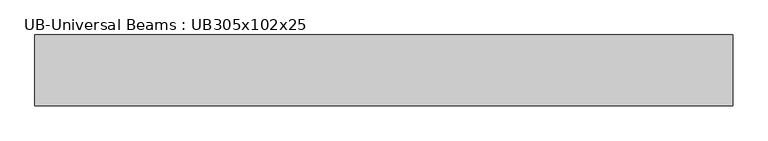
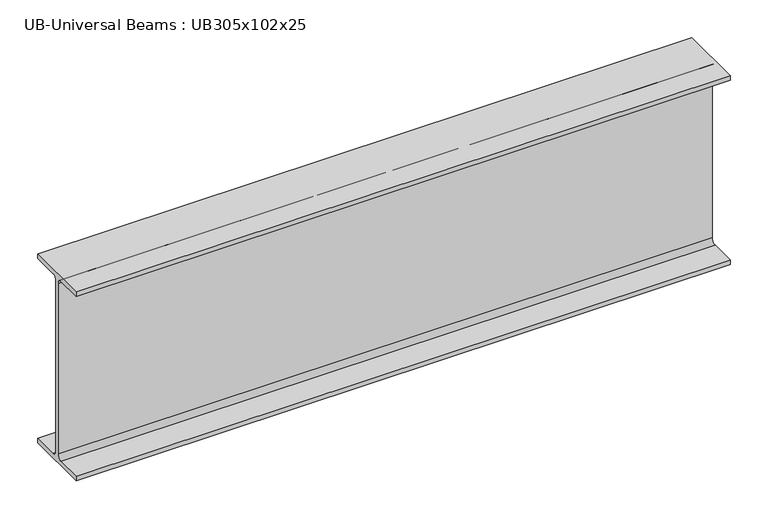
"""IFC4 building model written with IfcOpenShell, lengths in millimetres: beam geometry, UB-Universal Beams : UB305x102x25."""

import ifcopenshell
import ifcopenshell.guid

model = None  # the IFC model being written
_history = None  # IfcOwnerHistory: only IFC2X3 demands one
_inside = {}  # id of a spatial element -> (the spatial element, [elements in it])
_under = {}  # id of a project, library or spatial element -> (it, [spatial elements below it])
_declared = {}  # id of a project -> (the project, [libraries it declares])
_typed = {}  # id of a type object -> (the type object, [elements of that type])
_made_of = {}  # id of a material, layer set ... -> (it, [elements and type objects made of it])


def new_model(schema):
    """Start an empty IFC model of exactly this schema.

    Asked for "IFC4X3", IfcOpenShell would pick the latest addendum, in which some entities
    have other attributes; the version numbers below select the first issue.
    IFC2X3 requires an IfcOwnerHistory on every rooted entity: one is made here for all.
    """
    global model, _history
    if schema == "IFC4X3":
        model = ifcopenshell.file(schema_version=(4, 3, 0, 0))
    else:
        model = ifcopenshell.file(schema=schema)
    _inside.clear()
    _under.clear()
    _declared.clear()
    _typed.clear()
    _made_of.clear()
    _history = None
    if model.schema == "IFC2X3":
        org = make("IfcOrganization", Name="unknown")
        user = make(
            "IfcPersonAndOrganization",
            ThePerson=make("IfcPerson", FamilyName="unknown"),
            TheOrganization=org,
        )
        app = make(
            "IfcApplication",
            ApplicationDeveloper=org,
            Version="unknown",
            ApplicationFullName="unknown",
            ApplicationIdentifier="unknown",
        )
        _history = make(
            "IfcOwnerHistory",
            OwningUser=user,
            OwningApplication=app,
            ChangeAction="ADDED",
            CreationDate=0,
        )
    return model


def make(cls, **values):
    """One entity of the class cls with the attributes given. An attribute that is None is left unset."""
    return model.create_entity(
        cls, **{name: value for name, value in values.items() if value is not None}
    )


def rooted(cls, **values):
    """An entity with a GlobalId (a new one), such as an element, a storey or a relation."""
    return make(cls, GlobalId=ifcopenshell.guid.new(), OwnerHistory=_history, **values)


def si_unit(unit_type, name, prefix=None):
    """IfcSIUnit, for example si_unit("LENGTHUNIT", "METRE", prefix="MILLI")."""
    return make("IfcSIUnit", UnitType=unit_type, Prefix=prefix, Name=name)


def assignment(units):
    """IfcUnitAssignment: the units of a project."""
    return None if units is None else make("IfcUnitAssignment", Units=units)


def point(xyz):
    """IfcCartesianPoint."""
    return None if xyz is None else make("IfcCartesianPoint", Coordinates=xyz)


def direction(xyz):
    """IfcDirection."""
    return None if xyz is None else make("IfcDirection", DirectionRatios=xyz)


def frame(location, z_axis=None, x_axis=None):
    """IfcAxis2Placement3D, a coordinate frame: its origin and axes. An axis left out is left unset."""
    return make(
        "IfcAxis2Placement3D",
        Location=point(location),
        Axis=direction(z_axis),
        RefDirection=direction(x_axis),
    )


def frame_2d(location, x_axis=None):
    """IfcAxis2Placement2D, a coordinate frame in the plane: its origin and x axis."""
    return make(
        "IfcAxis2Placement2D", Location=point(location), RefDirection=direction(x_axis)
    )


def origin():
    """The frame at (0, 0, 0) with its axes left unset."""
    return frame((0.0, 0.0, 0.0))


def place(relative_to, where):
    """IfcLocalPlacement: puts the frame where relative to a parent placement (None: the world)."""
    return make(
        "IfcLocalPlacement", PlacementRelTo=relative_to, RelativePlacement=where
    )


def context(
    kind, dimensions, precision=None, world=None, true_north=None, identifier=None
):
    """IfcGeometricRepresentationContext, for example the 3D "Model" context."""
    return make(
        "IfcGeometricRepresentationContext",
        ContextIdentifier=identifier,
        ContextType=kind,
        CoordinateSpaceDimension=dimensions,
        Precision=precision,
        WorldCoordinateSystem=world,
        TrueNorth=true_north,
    )


def project(units=None, contexts=None):
    """IfcProject with its units and contexts."""
    return rooted(
        "IfcProject",
        Name="project",
        RepresentationContexts=contexts,
        UnitsInContext=assignment(units),
    )


def spatial(cls, under=None, at=None, **own):
    """A site, building, storey or space (cls), placed at a placement, below another one or the project."""
    s = rooted(cls, ObjectPlacement=at, **own)
    if under is not None:
        _under.setdefault(under.id(), (under, []))[1].append(s)
    return s


def polyline(points):
    """IfcPolyline through the points."""
    return make("IfcPolyline", Points=[point(p) for p in points])


def circle_curve(where, radius):
    """IfcCircle in the frame where."""
    return make("IfcCircle", Position=where, Radius=radius)


def trimmed(basis, trim1, trim2, sense, master):
    """IfcTrimmedCurve: the piece of a basis curve between two trims."""
    return make(
        "IfcTrimmedCurve",
        BasisCurve=basis,
        Trim1=trim1,
        Trim2=trim2,
        SenseAgreement=sense,
        MasterRepresentation=master,
    )


def segment(curve, same_sense, transition):
    """IfcCompositeCurveSegment."""
    return make(
        "IfcCompositeCurveSegment",
        Transition=transition,
        SameSense=same_sense,
        ParentCurve=curve,
    )


def composite_curve(segments, self_intersect=None):
    """IfcCompositeCurve: segments joined end to end."""
    return make("IfcCompositeCurve", Segments=segments, SelfIntersect=self_intersect)


def outline(outer, holes=None, kind="AREA"):
    """IfcArbitraryClosedProfileDef: a profile drawn as a closed curve; with holes, ...WithVoids."""
    if holes is None:
        return make("IfcArbitraryClosedProfileDef", ProfileType=kind, OuterCurve=outer)
    return make(
        "IfcArbitraryProfileDefWithVoids",
        ProfileType=kind,
        OuterCurve=outer,
        InnerCurves=holes,
    )


def extrude(swept, where, along, depth):
    """IfcExtrudedAreaSolid: the profile swept, set in the frame where, extruded along a direction by depth."""
    return make(
        "IfcExtrudedAreaSolid",
        SweptArea=swept,
        Position=where,
        ExtrudedDirection=direction(along),
        Depth=depth,
    )


def shape(context_of_items, identifier, shape_type, items):
    """IfcShapeRepresentation: the items that make up one representation, for example the "Body"."""
    return make(
        "IfcShapeRepresentation",
        ContextOfItems=context_of_items,
        RepresentationIdentifier=identifier,
        RepresentationType=shape_type,
        Items=items,
    )


def source(mapping_origin, context_of_items, identifier, shape_type, items):
    """IfcRepresentationMap: a shape defined once, which mapped items show again and again."""
    return make(
        "IfcRepresentationMap",
        MappingOrigin=mapping_origin,
        MappedRepresentation=shape(context_of_items, identifier, shape_type, items),
    )


def transform(
    local_origin,
    x_axis=None,
    y_axis=None,
    z_axis=None,
    scale=None,
    scale2=None,
    scale3=None,
    uniform=True,
):
    """IfcCartesianTransformationOperator3D, or its non-uniform kind. x_axis, y_axis, z_axis: its Axis1, 2, 3."""
    if uniform:
        return make(
            "IfcCartesianTransformationOperator3D",
            Axis1=direction(x_axis),
            Axis2=direction(y_axis),
            LocalOrigin=point(local_origin),
            Scale=scale,
            Axis3=direction(z_axis),
        )
    return make(
        "IfcCartesianTransformationOperator3DnonUniform",
        Axis1=direction(x_axis),
        Axis2=direction(y_axis),
        LocalOrigin=point(local_origin),
        Scale=scale,
        Axis3=direction(z_axis),
        Scale2=scale2,
        Scale3=scale3,
    )


def mapped(mapping_source, mapping_target):
    """IfcMappedItem: shows the shape of a source again, moved by a transform."""
    return make(
        "IfcMappedItem", MappingSource=mapping_source, MappingTarget=mapping_target
    )


def made_of(thing, what):
    """Note that an element or type object is made of a material, layer set ...; save() writes the relation."""
    if what is not None:
        _made_of.setdefault(what.id(), (what, []))[1].append(thing)
    return thing


def element(
    cls,
    number,
    at=None,
    inside=None,
    cuts=None,
    type_object=None,
    material=None,
    context=None,
    identifier="Body",
    shape_type=None,
    held_by="IfcProductDefinitionShape",
    body=None,
    shapes=None,
    **own,
):
    """One element of the class cls, such as IfcWall. Its Tag is "e" and its number.

    at: its placement. inside: the storey or other place that contains it. cuts: it is an
    opening in that element (IfcRelVoidsElement). A single representation is given by context,
    identifier, shape_type and body (its items); several are given by shapes. held_by: the class
    of the entity that holds the representations. save() writes the other relations.
    """
    e = rooted(cls, Tag="e%d" % number, ObjectPlacement=at, **own)
    if body is not None:
        shapes = [shape(context, identifier, shape_type, body)]
    if shapes is not None:
        e.Representation = make(held_by, Representations=shapes)
    if inside is not None:
        _inside.setdefault(inside.id(), (inside, []))[1].append(e)
    if cuts is not None:
        rooted(
            "IfcRelVoidsElement", RelatingBuildingElement=cuts, RelatedOpeningElement=e
        )
    if type_object is not None:
        _typed.setdefault(type_object.id(), (type_object, []))[1].append(e)
    return made_of(e, material)


def aggregate(whole, parts):
    """IfcRelAggregates: a whole, such as a stair, and the parts it consists of."""
    return rooted("IfcRelAggregates", RelatingObject=whole, RelatedObjects=parts)


def save(model, path):
    """Write the relations noted so far, then the file.

    IfcRelAggregates (storeys below a building ...), IfcRelContainedInSpatialStructure (elements
    in a storey), IfcRelDefinesByType, IfcRelAssociatesMaterial and IfcRelDeclares: one each for
    every whole, place, type object, material and project.
    """
    for whole, parts in _under.values():
        aggregate(whole, parts)
    for where, things in _inside.values():
        rooted(
            "IfcRelContainedInSpatialStructure",
            RelatedElements=things,
            RelatingStructure=where,
        )
    for kind, things in _typed.values():
        rooted("IfcRelDefinesByType", RelatedObjects=things, RelatingType=kind)
    for what, things in _made_of.values():
        rooted("IfcRelAssociatesMaterial", RelatedObjects=things, RelatingMaterial=what)
    for by, libraries in _declared.values():
        rooted("IfcRelDeclares", RelatingContext=by, RelatedDefinitions=libraries)
    model.write(path)


def ub_universal_beams_ub305x102x25_41277c4d(model_context):
    return source(origin(), model_context, "Body", "SweptSolid", [
        extrude(outline(composite_curve([segment(polyline([(50.8, -145.55), (50.8, -152.55), (-50.8, -152.55), (-50.8, -145.55), (-10.5, -145.55)]), True, "CONTINUOUS"), segment(trimmed(circle_curve(frame_2d((-10.5, -137.95)), 7.6), [point((-10.5, -145.55))], [point((-2.9, -137.95))], True, "CARTESIAN"), True, "CONTINUOUS"), segment(polyline([(-2.9, -137.95), (-2.9, 137.95)]), True, "CONTINUOUS"), segment(trimmed(circle_curve(frame_2d((-10.5, 137.95)), 7.6), [point((-2.9, 137.95))], [point((-10.5, 145.55))], True, "CARTESIAN"), True, "CONTINUOUS"), segment(polyline([(-10.5, 145.55), (-50.8, 145.55), (-50.8, 152.55), (50.8, 152.55), (50.8, 145.55), (10.5, 145.55)]), True, "CONTINUOUS"), segment(trimmed(circle_curve(frame_2d((10.5, 137.95)), 7.6), [point((10.5, 145.55))], [point((2.9, 137.95))], True, "CARTESIAN"), True, "CONTINUOUS"), segment(polyline([(2.9, 137.95), (2.9, -137.95)]), True, "CONTINUOUS"), segment(trimmed(circle_curve(frame_2d((10.5, -137.95)), 7.6), [point((2.9, -137.95))], [point((10.5, -145.55))], True, "CARTESIAN"), True, "CONTINUOUS"), segment(polyline([(10.5, -145.55), (50.8, -145.55)]), True, "CONTINUOUS")], self_intersect=False)), frame((-500.0, 0.0, 0.0), z_axis=(1.0, 0.0, 0.0), x_axis=(0.0, 1.0, 0.0)), (0.0, 0.0, 1.0), 1000.0),
    ])


if __name__ == "__main__":
    model = new_model("IFC4")
    model_context = context("Model", 3, world=origin())
    ifc_project = project(units=[si_unit("LENGTHUNIT", "METRE", prefix="MILLI")], contexts=[model_context])
    site = spatial("IfcSite", under=ifc_project)
    building = spatial("IfcBuilding", under=site)
    placement = place(None, origin())
    ub_universal_beams_ub305x102x25_shape = ub_universal_beams_ub305x102x25_41277c4d(model_context)
    element("IfcBeam", 1, ObjectType="UB-Universal Beams : UB305x102x25", at=placement, inside=building, context=model_context, shape_type="MappedRepresentation", body=[
        mapped(ub_universal_beams_ub305x102x25_shape, transform((0.0, 0.0, 0.0), x_axis=(1.0, 0.0, 0.0), y_axis=(0.0, 1.0, 0.0), z_axis=(0.0, 0.0, 1.0))),
    ])
    save(model, "model.ifc")

# Revit data of these elements
# Type "UB-Universal Beams : UB305x102x25"
#   Section Name Key = "UB305X102X25"
#   Width = 10.16 cm
#   Web Thickness = 0.58 cm
#   Web Fillet = 0.76 cm
#   Warping Constant = 27300.0 cm⁶
#   Torsional Moment of Inertia = 4.77 cm⁴
#   Section Area = 31.6 cm²
#   Plastic Modulus weak axis = 39.0 cm³
#   Plastic Modulus strong axis = 342.0 cm³
#   Nominal Weight = 24.7999 kgf/m
#   Moment of Inertia weak axis = 123.00 cm⁴
#   Moment of Inertia strong axis = 4455.00 cm⁴
#   Height = 30.51 cm
#   Flange Thickness = 0.7 cm
#   Elastic Modulus weak axis = 24.2 cm³
#   Elastic Modulus strong axis = 292.0 cm³
#   Centroid Vertical = 15.255 cm
#   Centroid Horizontal = 5.08 cm
#   Length [instance default] = 1500 mm
#   Structural Material [instance default] = Metal - Steel 43-275
#   Type Comments = ""
#   Assembly Code = ""
# Element 1 (IfcBeam, "UB-Universal Beams : UB305x102x25")
#   Structural Material = Metal - Steel
#   Materials on its faces: "Metal - Steel"
# Materials
#   "Metal - Steel 43-275": class "Metal", colour RGB 255 128 0, transparency 0, Cost = 0
#   "Metal - Steel": class "Metal", colour RGB 255 128 0, transparency 0, Cost = 0
